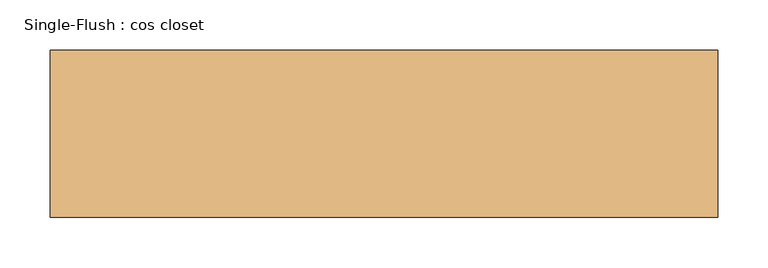
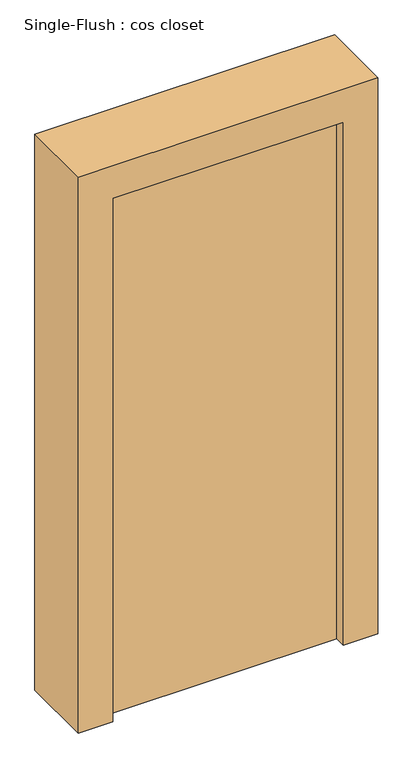
"""IFC4 building model written with IfcOpenShell, lengths in millimetres: door geometry, Single-Flush : cos closet."""

from ifc_helpers import new_model, si_unit, frame, origin, origin_with_axes, place, context, project, spatial, polyline, outline, extrude, source, transform, mapped, element, save


def single_flush_cos_closet_50bca49d(model_context):
    return source(origin(), model_context, "Body", "SweptSolid", [
        extrude(outline(polyline([(1295.4, 330.2), (1295.4, -330.2), (0.0, -330.2), (0.0, -254.0), (1219.2, -254.0), (1219.2, 254.0), (0.0, 254.0), (0.0, 330.2), (1295.4, 330.2)])), frame((0.0, -82.55, 0.0), z_axis=(0.0, 1.0, 0.0), x_axis=(0.0, 0.0, 1.0)), (0.0, 0.0, 1.0), 165.1),
        extrude(outline(polyline([(254.0, -6.35), (254.0, -57.15), (-254.0, -57.15), (-254.0, -6.35), (254.0, -6.35)])), origin_with_axes(), (0.0, 0.0, 1.0), 1219.2),
    ])


if __name__ == "__main__":
    model = new_model("IFC4")
    model_context = context("Model", 3, world=origin())
    ifc_project = project(units=[si_unit("LENGTHUNIT", "METRE", prefix="MILLI")], contexts=[model_context])
    site = spatial("IfcSite", under=ifc_project)
    building = spatial("IfcBuilding", under=site)
    placement = place(None, origin())
    single_flush_cos_closet_shape = single_flush_cos_closet_50bca49d(model_context)
    element("IfcDoor", 1, ObjectType="Single-Flush : cos closet", at=placement, inside=building, context=model_context, shape_type="MappedRepresentation", body=[
        mapped(single_flush_cos_closet_shape, transform((0.0, 0.0, 0.0), x_axis=(1.0, 0.0, 0.0), y_axis=(0.0, 1.0, 0.0), z_axis=(0.0, 0.0, 1.0))),
    ])
    save(model, "model.ifc")

# Revit data of these elements
# Type "Single-Flush : cos closet"
#   Type Mark = "68"
#   OD_DS_Door_Material = "T.B.D."
#   OD_DS_Door_Type = "SWING"
#   OD_DS_Lockset = "PRIVACY LOCK"
#   Assembly Code = "C1020"
#   Analytic Construction = "<None>"
#   Thickness = 0' - 2"
#   RO Offset = 0' - 0 1/4"
#   Height = 4' - 0"
#   Trim Projection Ext = 0' - 1"
#   Trim Projection Int = 0' - 1"
#   Trim Width = 0' - 3"
#   Width = 1' - 8"
#   Door Material = Closet_1
#   Frame Material = Closet_1
#   Function = (empty or 0)
#   Wall Closure = (empty or 0)
# Element 1 (IfcDoor, "Single-Flush : cos closet")
#   Materials on its faces: "Closet_1"
# Materials
#   "Closet_1": class "Paint", colour RGB 200 194 183, transparency 0, Cost = 0
